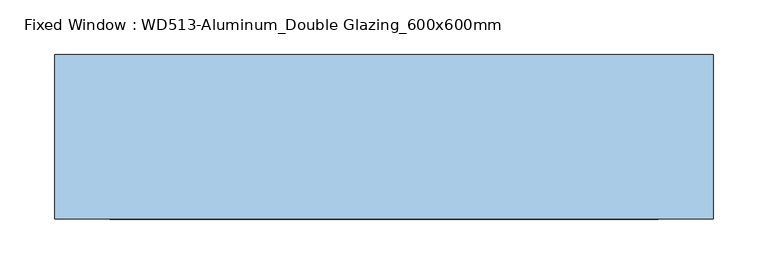
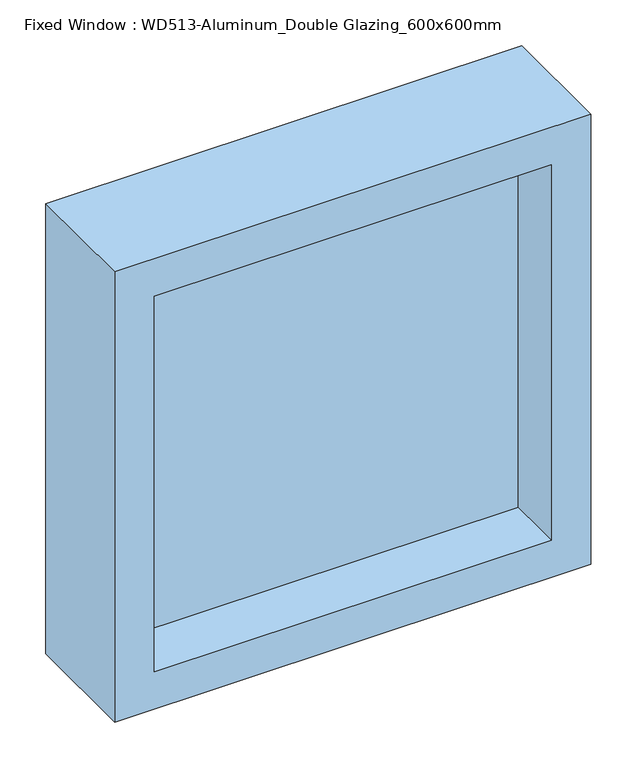
"""IFC4 building model written with IfcOpenShell, lengths in millimetres: window geometry, Fixed Window : WD513-Aluminum_Double Glazing_600x600mm."""

from ifc_helpers import new_model, si_unit, frame, origin, place, context, project, spatial, polyline, outline, extrude, source, transform, mapped, element, save


def fixed_window_wd513_aluminum_double_glazing_600x600mm_33f90cc5(model_context):
    return source(origin(), model_context, "Body", "SweptSolid", [
        extrude(outline(polyline([(-250.0, 3.0), (250.0, 3.0), (250.0, -3.0), (-250.0, -3.0), (-250.0, 3.0)])), frame((0.0, 0.0, 850.0), z_axis=(0.0, 0.0, 1.0), x_axis=(1.0, 0.0, 0.0)), (0.0, 0.0, 1.0), 500.0),
        extrude(outline(polyline([(1400.0, -300.0), (800.0, -300.0), (800.0, 300.0), (1400.0, 300.0), (1400.0, -300.0)]), holes=[polyline([(1350.0, -250.0), (1350.0, 250.0), (850.0, 250.0), (850.0, -250.0), (1350.0, -250.0)])]), frame((0.0, -75.0, 0.0), z_axis=(0.0, 1.0, 0.0), x_axis=(0.0, 0.0, 1.0)), (0.0, 0.0, 1.0), 150.0),
    ])


if __name__ == "__main__":
    model = new_model("IFC4")
    model_context = context("Model", 3, world=origin())
    ifc_project = project(units=[si_unit("LENGTHUNIT", "METRE", prefix="MILLI")], contexts=[model_context])
    site = spatial("IfcSite", under=ifc_project)
    building = spatial("IfcBuilding", under=site)
    placement = place(None, origin())
    fixed_window_wd513_aluminum_double_glazing_600x600mm_shape = fixed_window_wd513_aluminum_double_glazing_600x600mm_33f90cc5(model_context)
    element("IfcWindow", 1, ObjectType="Fixed Window : WD513-Aluminum_Double Glazing_600x600mm", at=placement, inside=building, context=model_context, shape_type="MappedRepresentation", body=[
        mapped(fixed_window_wd513_aluminum_double_glazing_600x600mm_shape, transform((0.0, 0.0, 0.0), x_axis=(1.0, 0.0, 0.0), y_axis=(0.0, 1.0, 0.0), z_axis=(0.0, 0.0, 1.0))),
    ])
    save(model, "model.ifc")

# Revit data of these elements
# Type "Fixed Window : WD513-Aluminum_Double Glazing_600x600mm"
#   Type Mark = "196"
#   Analytic Construction = "<None>"
#   창 두께 = 150 mm
#   Height = 600 mm
#   절반 창 두께 = 75 mm
#   기본 씰 높이 = 800 mm
#   Width = 600 mm
#   Define Thermal Properties by = 1
#   창 패널 = AW2 창 패널
#   창 프레임 = A04AQ127-00002_Aluminum Window_None FP
#   Wall Closure = (empty or 0)
# Element 1 (IfcWindow, "Fixed Window : WD513-Aluminum_Double Glazing_600x600mm")
#   Materials on its faces: "A04AQ127-00002_Aluminum Window_None FP", "AW2 창 패널"
# Materials
#   "AW2 창 패널": class "유리", colour RGB 0 0 255, transparency 0.75
#   "A04AQ127-00002_Aluminum Window_None FP": class "금속", colour RGB 247 247 247, transparency 0, W00) Work Master Code = "A04AQ127-00002", W01) Work Master_Lv1 = "Finishing Work", W02) Work Master_Lv2 = "Door & Window Work", W03) Work Master_Spec.1 = "Aluminum Window", W04) Work Master_Spec.2 = "Fire Protective Rating: N/A", W05) Work Master_Spec.3 = "w/ Hardware & Accessories", Cost = 0
